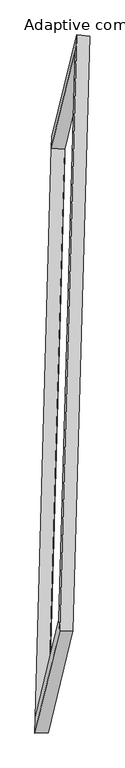
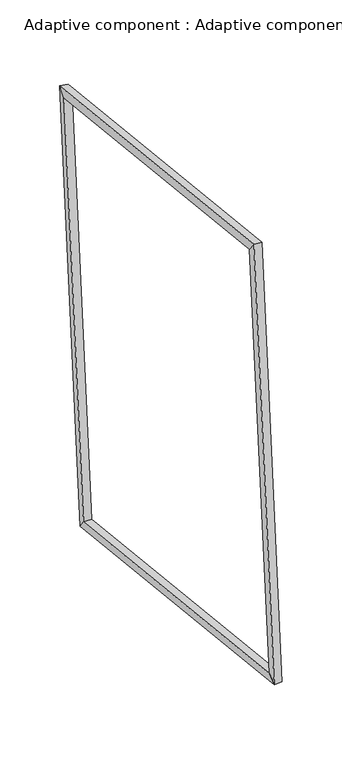
"""IFC4 building model written with IfcOpenShell, lengths in millimetres: proxy geometry, Adaptive component : Adaptive component."""

from ifc_helpers import new_model, si_unit, origin, place, context, project, spatial, faceted_brep, source, transform, mapped, element, save


def adaptive_component_adaptive_component_6756c52a(model_context):
    return source(origin(), model_context, "Body", "Brep", [
        faceted_brep([(73.8297174, 1205.2681046, 2815.4458577), (138.4728494, 1199.3759905, 2810.6905876), (59.5627198, -1565.3624951, 3209.0288681), (-5.2682713, -1566.0523156, 3214.7324508), (81.2075304, 1278.5743736, 2870.3156553), (-1.5566733, -1621.1975608, 3288.1092991), (145.8506624, 1272.6822595, 2865.5603852), (63.2743178, -1620.5077403, 3282.4057164), (-55.666274, -2041.9856426, -121.886484), (-120.7249481, -2043.6172316, -122.7645184), (-121.4567608, -2117.1418125, -177.8329879), (-56.3980866, -2115.5102235, -176.9549536), (23.2438556, 722.7528431, -520.2247645), (-41.6269594, 727.7031887, -522.0511115), (-38.6925571, 782.6301219, -595.6266318), (26.1782579, 777.6797763, -593.8002847)], [[[0, 1, 2, 3]], [[4, 0, 3, 5]], [[6, 4, 5, 7]], [[1, 6, 7, 2]], [[3, 2, 8, 9]], [[5, 3, 9, 10]], [[7, 5, 10, 11]], [[2, 7, 11, 8]], [[9, 8, 12, 13]], [[10, 9, 13, 14]], [[11, 10, 14, 15]], [[8, 11, 15, 12]], [[13, 12, 1, 0]], [[14, 13, 0, 4]], [[15, 14, 4, 6]], [[12, 15, 6, 1]]]),
    ])


if __name__ == "__main__":
    model = new_model("IFC4")
    model_context = context("Model", 3, world=origin())
    ifc_project = project(units=[si_unit("LENGTHUNIT", "METRE", prefix="MILLI")], contexts=[model_context])
    site = spatial("IfcSite", under=ifc_project)
    building = spatial("IfcBuilding", under=site)
    placement = place(None, origin())
    adaptive_component_adaptive_component_shape = adaptive_component_adaptive_component_6756c52a(model_context)
    element("IfcBuildingElementProxy", 1, Name="Adaptive component : Adaptive component", ObjectType="Adaptive component : Adaptive component", at=placement, inside=building, context=model_context, shape_type="MappedRepresentation", body=[
        mapped(adaptive_component_adaptive_component_shape, transform((0.0, 0.0, 0.0), x_axis=(1.0, 0.0, 0.0), y_axis=(0.0, 1.0, 0.0), z_axis=(0.0, 0.0, 1.0))),
    ])
    save(model, "model.ifc")

# Revit data of these elements
# Type "Adaptive component : Adaptive component"
#   r [instance default] = 2063.125 mm
#   2r [instance default] = 4126.251 mm
#   Number [instance default] = 5
#   Default Elevation = 0
# Element 1 (IfcBuildingElementProxy, "Adaptive component : Adaptive component")
#   r = 2281.489 mm
#   2r = 4562.977 mm
#   Number = 13
